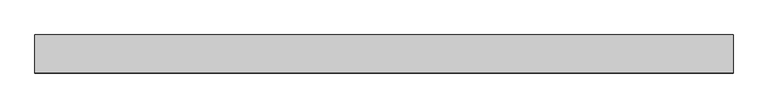
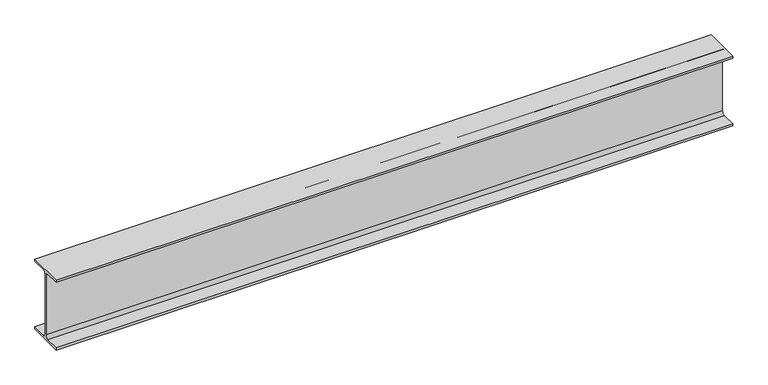
"""IFC4 building model written with IfcOpenShell, lengths in millimetres: beam geometry, Steel Framing_H_KS : H_SB_AR_S02_H-300x150x6.5x9_WG1."""

from ifc_helpers import new_model, si_unit, point, frame, frame_2d, origin, place, context, project, spatial, polyline, circle_curve, trimmed, segment, composite_curve, outline, extrude, source, transform, mapped, element, save


def beam_2976cc55(model_context):
    return source(origin(), model_context, "Body", "SweptSolid", [
        extrude(outline(composite_curve([segment(polyline([(-75.0, -141.0), (-16.25, -141.0)]), True, "CONTINUOUS"), segment(trimmed(circle_curve(frame_2d((-16.25, -128.0)), 13.0), [point((-16.25, -141.0))], [point((-3.25, -128.0))], True, "CARTESIAN"), True, "CONTINUOUS"), segment(polyline([(-3.25, -128.0), (-3.25, 128.0)]), True, "CONTINUOUS"), segment(trimmed(circle_curve(frame_2d((-16.25, 128.0)), 13.0), [point((-3.25, 128.0))], [point((-16.25, 141.0))], True, "CARTESIAN"), True, "CONTINUOUS"), segment(polyline([(-16.25, 141.0), (-75.0, 141.0), (-75.0, 150.0), (75.0, 150.0), (75.0, 141.0), (16.25, 141.0)]), True, "CONTINUOUS"), segment(trimmed(circle_curve(frame_2d((16.25, 128.0)), 13.0), [point((16.25, 141.0))], [point((3.25, 128.0))], True, "CARTESIAN"), True, "CONTINUOUS"), segment(polyline([(3.25, 128.0), (3.25, -128.0)]), True, "CONTINUOUS"), segment(trimmed(circle_curve(frame_2d((16.25, -128.0)), 13.0), [point((3.25, -128.0))], [point((16.25, -141.0))], True, "CARTESIAN"), True, "CONTINUOUS"), segment(polyline([(16.25, -141.0), (75.0, -141.0), (75.0, -150.0), (-75.0, -150.0), (-75.0, -141.0)]), True, "CONTINUOUS")], self_intersect=False)), frame((-1412.3, 0.0, 0.0), z_axis=(1.0, 0.0, 0.0), x_axis=(0.0, 1.0, 0.0)), (0.0, 0.0, 1.0), 2749.6),
    ])


if __name__ == "__main__":
    model = new_model("IFC4")
    model_context = context("Model", 3, world=origin())
    ifc_project = project(units=[si_unit("LENGTHUNIT", "METRE", prefix="MILLI")], contexts=[model_context])
    site = spatial("IfcSite", under=ifc_project)
    building = spatial("IfcBuilding", under=site)
    placement = place(None, origin())
    beam_shape = beam_2976cc55(model_context)
    element("IfcBeam", 1, ObjectType="Steel Framing_H_KS : H_SB_AR_S02_H-300x150x6.5x9_WG1", at=placement, inside=building, context=model_context, shape_type="MappedRepresentation", body=[
        mapped(beam_shape, transform((0.0, 0.0, 0.0), x_axis=(1.0, 0.0, 0.0), y_axis=(0.0, 1.0, 0.0), z_axis=(0.0, 0.0, 1.0))),
    ])
    save(model, "model.ifc")

# Revit data of these elements
# Type "Steel Framing_H_KS : H_SB_AR_S02_H-300x150x6.5x9_WG1"
#   Type Comments = "MAIN"
#   Type Mark = "WG1"
#   H_SectionID = "H-300x150x6.5x9"
#   H_Ratio for Additional Steel Plate = 0.2
#   Width = 15.0 cm
#   Web Thickness = 0.65 cm
#   Web Fillet = 1.3 cm
#   Warping Constant = 107000.0 cm⁶
#   Torsional Moment of Inertia = 9.9539 cm⁴
#   Section Area = 46.78 cm²
#   Plastic Modulus weak axis = 105.0 cm³
#   Plastic Modulus strong axis = 542.0 cm³
#   Perimeter = 1.17 m²/m
#   Nominal Weight = 36.70 kgf/m
#   Moment of Inertia weak axis = 508.00 cm⁴
#   Moment of Inertia strong axis = 7210.00 cm⁴
#   Height = 30.0 cm
#   Flange Thickness = 0.9 cm
#   Elastic Modulus weak axis = 67.7 cm³
#   Elastic Modulus strong axis = 481.0 cm³
#   Centroid Vertical = 15.0 cm
#   Centroid Horizontal = 7.5 cm
#   Bolt Spacing = 8.89 cm
#   Length [instance default] = 1500 mm
#   Structural Material [instance default] = Steel, 45-345
#   Section Name Key = ""
#   Assembly Code = ""
# Element 1 (IfcBeam, "Steel Framing_H_KS : H_SB_AR_S02_H-300x150x6.5x9_WG1")
#   Materials on its faces: "Steel, 45-345"
# Materials
#   "Steel, 45-345": class "Metal", colour RGB 189 187 185, transparency 0, Description = "Steel 345 MPa", Cost = 0
